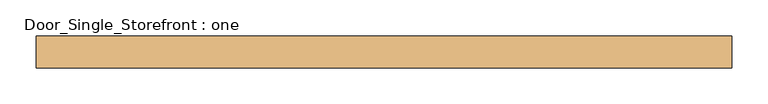
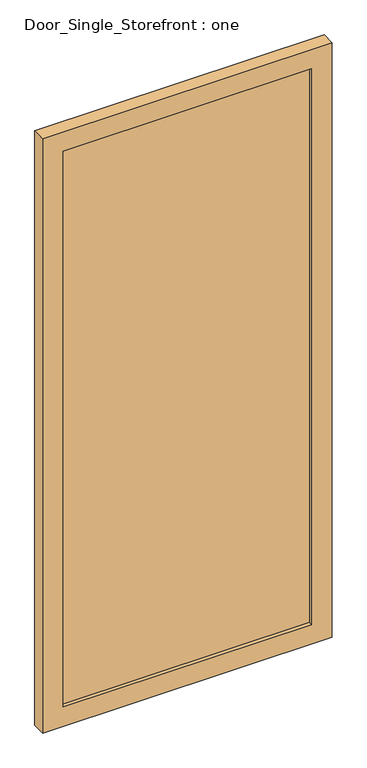
"""IFC4 building model written with IfcOpenShell, lengths in millimetres: door geometry, Door_Single_Storefront : one."""

from ifc_helpers import new_model, si_unit, frame, origin, place, context, project, spatial, polyline, outline, extrude, source, transform, mapped, element, save


def door_single_storefront_one_696d4805(model_context):
    return source(origin(), model_context, "Body", "SweptSolid", [
        extrude(outline(polyline([(414.734375, 6.35), (414.734375, -12.7), (-414.734375, -12.7), (-414.734375, 6.35), (414.734375, 6.35)])), frame((0.0, 0.0, 68.2625), z_axis=(0.0, 0.0, 1.0), x_axis=(1.0, 0.0, 0.0)), (0.0, 0.0, 1.0), 1958.975),
        extrude(outline(polyline([(2095.5, -482.996875), (0.0, -482.996875), (0.0, 482.996875), (2095.5, 482.996875), (2095.5, -482.996875)]), holes=[polyline([(68.2625, 414.734375), (68.2625, -414.734375), (2027.2375, -414.734375), (2027.2375, 414.734375), (68.2625, 414.734375)])]), frame((0.0, -25.4, 0.0), z_axis=(0.0, 1.0, 0.0), x_axis=(0.0, 0.0, 1.0)), (0.0, 0.0, 1.0), 44.45),
    ])


if __name__ == "__main__":
    model = new_model("IFC4")
    model_context = context("Model", 3, world=origin())
    ifc_project = project(units=[si_unit("LENGTHUNIT", "METRE", prefix="MILLI")], contexts=[model_context])
    site = spatial("IfcSite", under=ifc_project)
    building = spatial("IfcBuilding", under=site)
    placement = place(None, origin())
    door_single_storefront_one_shape = door_single_storefront_one_696d4805(model_context)
    element("IfcDoor", 1, ObjectType="Door_Single_Storefront : one", at=placement, inside=building, context=model_context, shape_type="MappedRepresentation", body=[
        mapped(door_single_storefront_one_shape, transform((0.0, 0.0, 0.0), x_axis=(1.0, 0.0, 0.0), y_axis=(0.0, 1.0, 0.0), z_axis=(0.0, 0.0, 1.0))),
    ])
    save(model, "model.ifc")

# Revit data of these elements
# Type "Door_Single_Storefront : one"
#   Type Mark = "29"
#   OD_DS_Door_Material = "ALUM./GLAZING"
#   OD_DS_Door_Type = "STOREFRONT (NARROW STILE)"
#   OD_DS_Lockset = "ENTRY LOCK (INSIDE ADA LEVER ALWAYS ACTIVE)"
#   Analytic Construction = "<None>"
#   angle open [instance default] = 132.952°
#   Stile_Width = 0' - 2 11/16"
#   Door_Thickness = 0' - 1 3/4"
#   Door_Offset = 0' - 1"
#   Glass_Material = TEMPERED INSULATED GLAZING (CARDINAL GLASS LoĒ²-240\nOR EQUIVALENT)
#   Frame_Material = KAWNEER 260 INSULCLADTM THERMAL ENTRANCE - CLEAR ANODIZED ALUM.
#   Function = (empty or 0)
# Element 1 (IfcDoor, "Door_Single_Storefront : one")
#   angle open = 170.00°
#   Materials on its faces: "KAWNEER 260 INSULCLADTM THERMAL ENTRANCE - CLEAR ANODIZED ALUM.", "TEMPERED INSULATED GLAZING (CARDINAL GLASS LoĒ²-240\nOR EQUIVALENT)"
# Materials
#   "TEMPERED INSULATED GLAZING (CARDINAL GLASS LoĒ²-240\nOR EQUIVALENT)": class "Glass", colour RGB 196 205 210, transparency 0.85, Description = "Soda Lime Glass", Cost = 0
#   "KAWNEER 260 INSULCLADTM THERMAL ENTRANCE - CLEAR ANODIZED ALUM.": class "Metal", colour RGB 244 244 244, transparency 0, Description = "Aluminum 6061", Cost = 0
